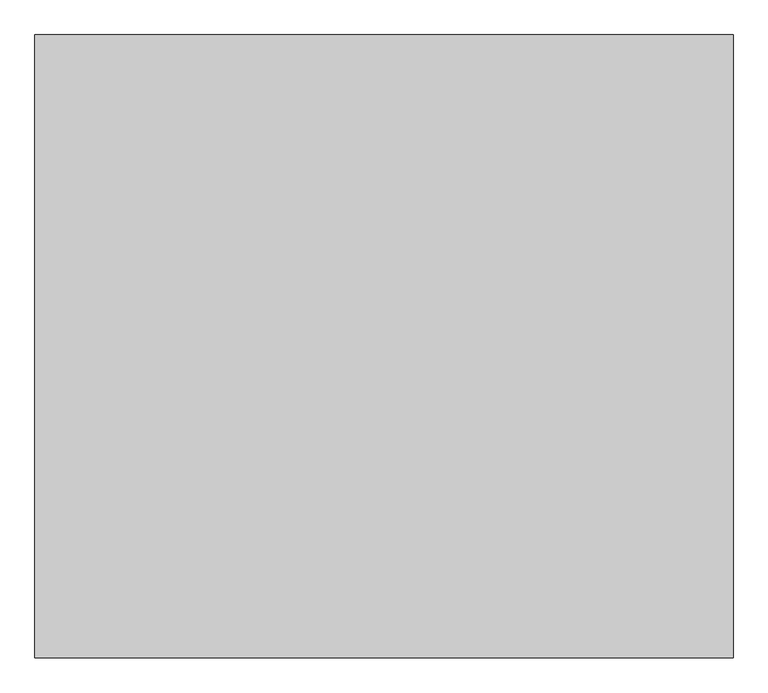
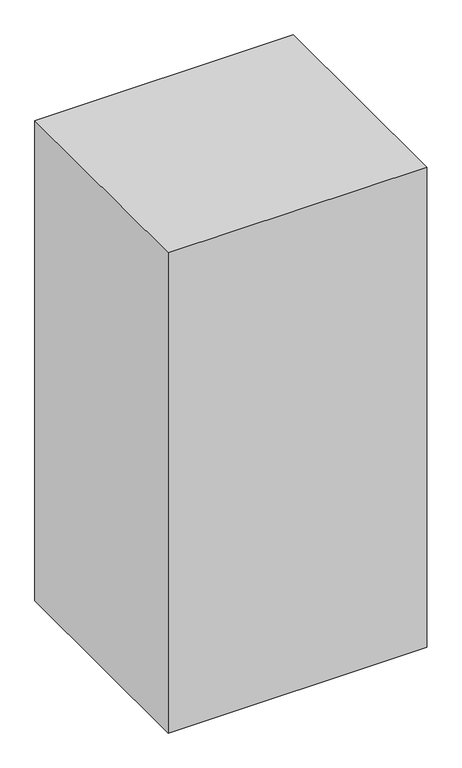
"""IFC4 building model written with IfcOpenShell, lengths in millimetres: proxy geometry, Space Planning Box_hec : Space Planning Box_hec."""

from ifc_helpers import new_model, si_unit, origin, origin_with_axes, place, context, project, spatial, polyline, outline, extrude, source, transform, mapped, element, save


def generic_models_0ee3397c(model_context):
    return source(origin(), model_context, "Body", "SweptSolid", [
        extrude(outline(polyline([(1400.0, 1250.0), (1400.0, -1250.0), (-1400.0, -1250.0), (-1400.0, 1250.0), (1400.0, 1250.0)])), origin_with_axes(), (0.0, 0.0, 1.0), 5500.0),
    ])


if __name__ == "__main__":
    model = new_model("IFC4")
    model_context = context("Model", 3, world=origin())
    ifc_project = project(units=[si_unit("LENGTHUNIT", "METRE", prefix="MILLI")], contexts=[model_context])
    site = spatial("IfcSite", under=ifc_project)
    building = spatial("IfcBuilding", under=site)
    placement = place(None, origin())
    generic_models_shape = generic_models_0ee3397c(model_context)
    element("IfcBuildingElementProxy", 1, Name="Space Planning Box_hec : Space Planning Box_hec", ObjectType="Space Planning Box_hec : Space Planning Box_hec", at=placement, inside=building, context=model_context, shape_type="MappedRepresentation", body=[
        mapped(generic_models_shape, transform((0.0, 0.0, 0.0), x_axis=(1.0, 0.0, 0.0), y_axis=(0.0, 1.0, 0.0), z_axis=(0.0, 0.0, 1.0))),
    ])
    save(model, "model.ifc")

# Revit data of these elements
# Type "Space Planning Box_hec : Space Planning Box_hec"
#   Type Comments = "..."
#   Room Name [instance default] = "?"
#   Interior Finish [instance default] = ""
#   Exterior Finish [instance default] = ""
#   Department [instance default] = ""
#   Assembly Code = "..."
#   ceiling height [instance default] = 0
#   Width [instance default] = 1524 mm
#   Program Area [instance default] = 0.00 m²
#   Length [instance default] = 1524 mm
#   Height [instance default] = 1524 mm
#   Area [instance default] = 2.32258 m²
#   Fill Color [instance default] = Cyan
#   Default Elevation = 0
# Element 1 (IfcBuildingElementProxy, "Space Planning Box_hec : Space Planning Box_hec")
#   Room Name = "Locker(F)"
#   Exterior Finish = "N/A..N/A,,N/A..N/A..N/A"
#   Department = "AR"
#   Width = 2800 mm
#   Program Area = 7.00 m²
#   Length = 2500 mm
#   Height = 5500 mm
#   Area = 7.00 m²
#   Materials on its faces: "Cyan"
# Materials
#   "Cyan": class "Generic", colour RGB 0 255 255, transparency 0.2, Cost = 0
